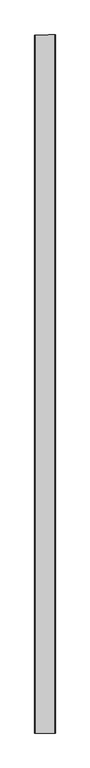
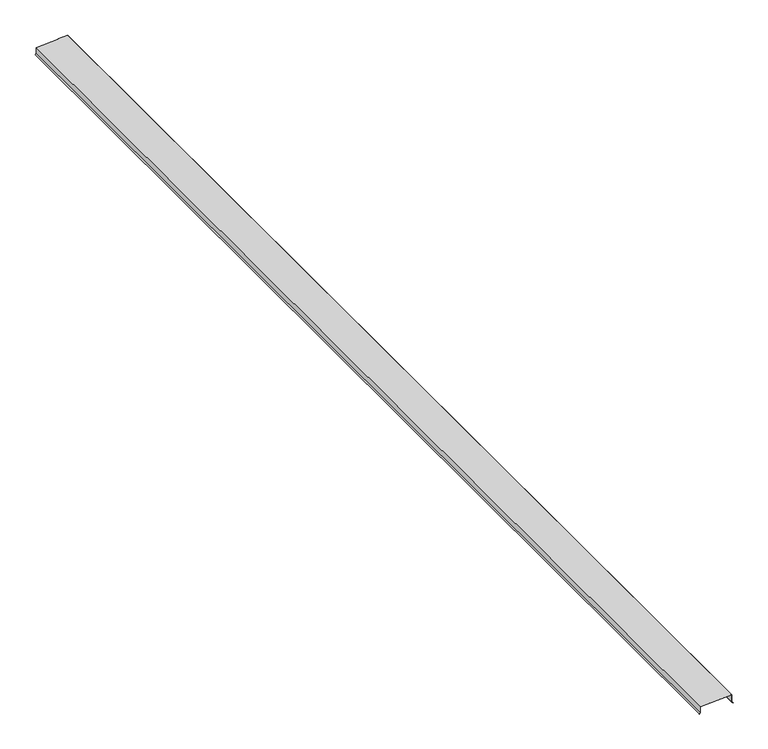
"""IFC4 building model written with IfcOpenShell, lengths in millimetres: proxy geometry, Generic Models 7:Generic Models 1:5:Generic Models 1:5 : Generic Models 7:Generic Models 1:337419:31 : Generic Models 7:Generic Models 1:5:Generic Models 1:5 : Generic Models 7:Generic Models 1:337419:311462."""

from ifc_helpers import new_model, si_unit, origin, place, context, project, spatial, faceted_brep, source, transform, mapped, element, save


def generic_models_ac987d50(model_context):
    return source(origin(), model_context, "Body", "Brep", [
        faceted_brep([(667671.1367239, -581169.2163841, 6087.1348677), (667658.4367239, -581169.2163841, 6099.8348677), (667658.4367239, -581169.2163841, 6188.1524863), (667301.2492239, -581169.2163841, 6169.4330826), (667301.2492239, -581169.2163841, 6099.8348677), (667288.5492239, -581169.2163841, 6087.1348677), (667289.6717559, -581169.2163841, 6086.0123357), (667302.8367239, -581169.2163841, 6099.1773037), (667302.8367239, -581169.2163841, 6167.9266014), (667656.8492239, -581169.2163841, 6186.4796103), (667656.8492239, -581169.2163841, 6099.1773037), (667670.0141919, -581169.2163841, 6086.0123357), (667658.4367239, -568233.850616, 6188.1524863), (667658.4367239, -568233.850616, 6099.8348677), (667671.1367239, -568233.850616, 6087.1348677), (667670.0141919, -568233.850616, 6086.0123357), (667656.8492239, -568233.850616, 6099.1773037), (667656.8492239, -568233.850616, 6186.4796103), (667548.8992239, -568233.850616, 6180.8221905), (667548.8992239, -568233.850616, 6182.4118691), (667302.8367239, -568236.4915363, 6167.9266014), (667548.8992239, -568236.4915363, 6180.8221905), (667302.8367239, -568236.4915363, 6099.1773037), (667289.6717559, -568236.4915363, 6086.0123357), (667288.5492239, -568236.4915363, 6087.1348677), (667301.2492239, -568236.4915363, 6099.8348677), (667301.2492239, -568236.4915363, 6169.4330826), (667548.8992239, -568236.4915363, 6182.4118691), (667547.3117239, -568236.4915363, 6182.3286718)], [[[0, 1, 2, 3, 4, 5, 6, 7, 8, 9, 10, 11]], [[12, 13, 14, 15, 16, 17, 18, 19]], [[1, 0, 14, 13]], [[0, 11, 15, 14]], [[11, 10, 16, 15]], [[10, 9, 17, 16]], [[9, 8, 20, 21, 18, 17]], [[8, 7, 22, 20]], [[7, 6, 23, 22]], [[6, 5, 24, 23]], [[5, 4, 25, 24]], [[4, 3, 26, 25]], [[3, 2, 12, 19, 27, 28, 26]], [[2, 1, 13, 12]], [[27, 21, 20, 22, 23, 24, 25, 26, 28]], [[21, 27, 19, 18]]]),
    ])


if __name__ == "__main__":
    model = new_model("IFC4")
    model_context = context("Model", 3, world=origin())
    ifc_project = project(units=[si_unit("LENGTHUNIT", "METRE", prefix="MILLI")], contexts=[model_context])
    site = spatial("IfcSite", under=ifc_project)
    building = spatial("IfcBuilding", under=site)
    placement = place(None, origin())
    generic_models_shape = generic_models_ac987d50(model_context)
    element("IfcBuildingElementProxy", 1, Name="Generic Models 7:Generic Models 1:5:Generic Models 1:5 : Generic Models 7:Generic Models 1:337419:31 : Generic Models 7:Generic Models 1:5:Generic Models 1:5 : Generic Models 7:Generic Models 1:337419:311462", ObjectType="Generic Models 7:Generic Models 1:5:Generic Models 1:5 : Generic Models 7:Generic Models 1:337419:31 : Generic Models 7:Generic Models 1:5:Generic Models 1:5 : Generic Models 7:Generic Models 1:337419:311462", at=placement, inside=building, context=model_context, shape_type="MappedRepresentation", body=[
        mapped(generic_models_shape, transform((0.0, 0.0, 0.0), x_axis=(1.0, 0.0, 0.0), y_axis=(0.0, 1.0, 0.0), z_axis=(0.0, 0.0, 1.0))),
    ])
    save(model, "model.ifc")

# Revit data of these elements
# Type "Generic Models 7:Generic Models 1:5:Generic Models 1:5 : Generic Models 7:Generic Models 1:337419:31 : Generic Models 7:Generic Models 1:5:Generic Models 1:5 : Generic Models 7:Generic Models 1:337419:311462"
#   NameOverride = "Generic Models 7:Generic Models 1:5:Generic Models 1:5 : Generic Models 7:Generic Models 1:337419:311462"
#   ObjectTypeOverride = "Generic Models 1:5 : Generic Models 7:Generic Models 1:337419"
#   Reference = "Generic Models 1"
#   Tag = "311462"
# Element 1 (IfcBuildingElementProxy, "Generic Models 7:Generic Models 1:5:Generic Models 1:5 : Generic Models 7:Generic Models 1:337419:31 : Generic Models 7:Generic Models 1:5:Generic Models 1:5 : Generic Models 7:Generic Models 1:337419:311462")
#   Materials on its faces: "SLOPED SHEET METAL COPING - (COLOR TO MATCH RESIN PANEL)"
# Materials
#   "SLOPED SHEET METAL COPING - (COLOR TO MATCH RESIN PANEL)": class "Generic", colour RGB 240 240 240, transparency 0, Keynote = "M07711300.01", Cost = 0
